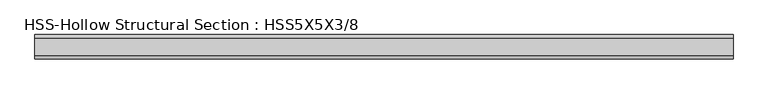
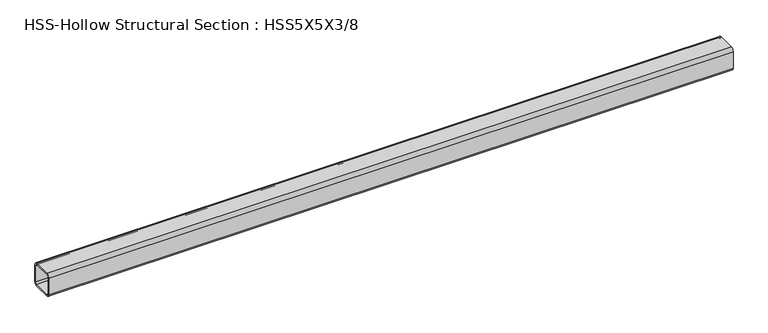
"""IFC4 building model written with IfcOpenShell, lengths in millimetres: beam geometry, HSS-Hollow Structural Section : HSS5X5X3/8."""

from ifc_helpers import new_model, si_unit, point, frame, frame_2d, origin, place, context, project, spatial, polyline, circle_curve, trimmed, segment, composite_curve, outline, extrude, source, transform, mapped, element, save


def hss_hollow_structural_section_hss5x5x3_8_b32892de(model_context):
    return source(origin(), model_context, "Body", "SweptSolid", [
        extrude(outline(composite_curve([segment(polyline([(63.5, 45.7708), (63.5, -45.7708)]), True, "CONTINUOUS"), segment(trimmed(circle_curve(frame_2d((45.7708, -45.7708)), 17.7292), [point((63.5, -45.7708))], [point((45.7708, -63.5))], False, "CARTESIAN"), True, "CONTINUOUS"), segment(polyline([(45.7708, -63.5), (-45.7708, -63.5)]), True, "CONTINUOUS"), segment(trimmed(circle_curve(frame_2d((-45.7708, -45.7708)), 17.7292), [point((-45.7708, -63.5))], [point((-63.5, -45.7708))], False, "CARTESIAN"), True, "CONTINUOUS"), segment(polyline([(-63.5, -45.7708), (-63.5, 45.7708)]), True, "CONTINUOUS"), segment(trimmed(circle_curve(frame_2d((-45.7708, 45.7708)), 17.7292), [point((-63.5, 45.7708))], [point((-45.7708, 63.5))], False, "CARTESIAN"), True, "CONTINUOUS"), segment(polyline([(-45.7708, 63.5), (45.7708, 63.5)]), True, "CONTINUOUS"), segment(trimmed(circle_curve(frame_2d((45.7708, 45.7708)), 17.7292), [point((45.7708, 63.5))], [point((63.5, 45.7708))], False, "CARTESIAN"), True, "CONTINUOUS")], self_intersect=False), holes=[composite_curve([segment(trimmed(circle_curve(frame_2d((-45.7708, 45.7708)), 8.8646), [point((-45.7708, 54.6354))], [point((-54.6354, 45.7708))], True, "CARTESIAN"), True, "CONTINUOUS"), segment(polyline([(-54.6354, 45.7708), (-54.6354, -45.7708)]), True, "CONTINUOUS"), segment(trimmed(circle_curve(frame_2d((-45.7708, -45.7708)), 8.8646), [point((-54.6354, -45.7708))], [point((-45.7708, -54.6354))], True, "CARTESIAN"), True, "CONTINUOUS"), segment(polyline([(-45.7708, -54.6354), (45.7708, -54.6354)]), True, "CONTINUOUS"), segment(trimmed(circle_curve(frame_2d((45.7708, -45.7708)), 8.8646), [point((45.7708, -54.6354))], [point((54.6354, -45.7708))], True, "CARTESIAN"), True, "CONTINUOUS"), segment(polyline([(54.6354, -45.7708), (54.6354, 45.7708)]), True, "CONTINUOUS"), segment(trimmed(circle_curve(frame_2d((45.7708, 45.7708)), 8.8646), [point((54.6354, 45.7708))], [point((45.7708, 54.6354))], True, "CARTESIAN"), True, "CONTINUOUS"), segment(polyline([(45.7708, 54.6354), (-45.7708, 54.6354)]), True, "CONTINUOUS")], self_intersect=False)]), frame((-1819.275, 0.0, 0.0), z_axis=(1.0, 0.0, 0.0), x_axis=(0.0, 1.0, 0.0)), (0.0, 0.0, 1.0), 3638.55),
    ])


if __name__ == "__main__":
    model = new_model("IFC4")
    model_context = context("Model", 3, world=origin())
    ifc_project = project(units=[si_unit("LENGTHUNIT", "METRE", prefix="MILLI")], contexts=[model_context])
    site = spatial("IfcSite", under=ifc_project)
    building = spatial("IfcBuilding", under=site)
    placement = place(None, origin())
    hss_hollow_structural_section_hss5x5x3_8_shape = hss_hollow_structural_section_hss5x5x3_8_b32892de(model_context)
    element("IfcBeam", 1, ObjectType="HSS-Hollow Structural Section : HSS5X5X3/8", at=placement, inside=building, context=model_context, shape_type="MappedRepresentation", body=[
        mapped(hss_hollow_structural_section_hss5x5x3_8_shape, transform((0.0, 0.0, 0.0), x_axis=(1.0, 0.0, 0.0), y_axis=(0.0, 1.0, 0.0), z_axis=(0.0, 0.0, 1.0))),
    ])
    save(model, "model.ifc")

# Revit data of these elements
# Type "HSS-Hollow Structural Section : HSS5X5X3/8"
#   Assembly Code = "B10"
#   Shape = "Square"
#   W = 22.3
#   Ht = 0' - 5"
#   Length [instance default] = 5' - 0"
#   b = 0' - 5"
#   kr = 0' - 0.698"
#   t = 0' - 0.349"
#   A = 0.0429167 SF
#   Structural Material [instance default] = Steel ASTM A500, Grade B, Rectangular and Square
# Element 1 (IfcBeam, "HSS-Hollow Structural Section : HSS5X5X3/8")
#   Materials on its faces: "Steel ASTM A500, Grade B, Rectangular and Square"
# Materials
#   "Steel ASTM A500, Grade B, Rectangular and Square": class "Metal", colour RGB 199 199 199, transparency 0, Description = "Carbon steel", Cost = 0
